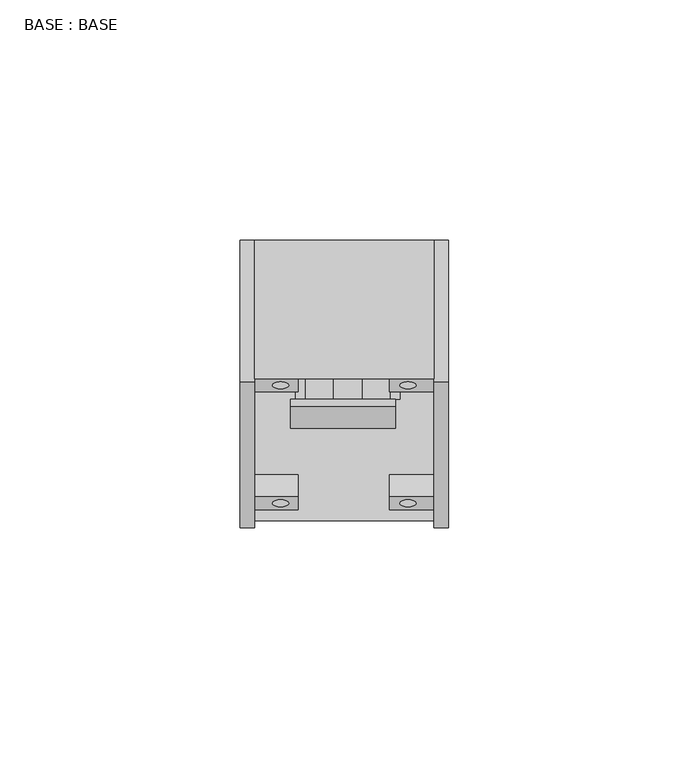
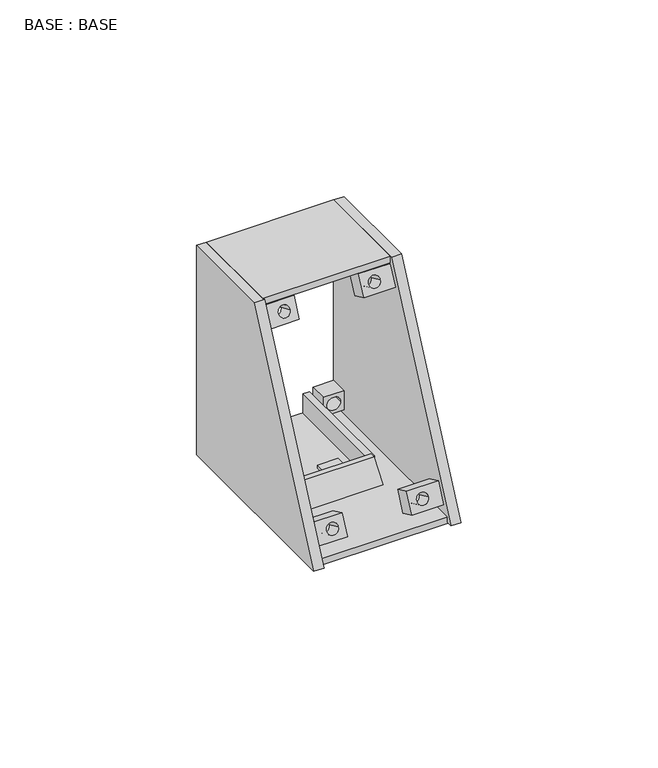
"""IFC4 building model written with IfcOpenShell, lengths in millimetres: proxy geometry, BASE : BASE."""

from ifc_helpers import new_model, si_unit, point, frame, frame_2d, origin, origin_with_axes, place, context, project, spatial, polyline, circle_curve, trimmed, segment, composite_curve, outline, extrude, source, transform, mapped, element, save


def base_base_dd735b77(model_context):
    return source(origin(), model_context, "Body", "SweptSolid", [
        extrude(outline(polyline([(3.2, -2.2), (-3.2, -2.2), (-3.2, 7.1), (3.2, 7.1), (3.2, -2.2)]), holes=[composite_curve([segment(trimmed(circle_curve(frame_2d((0.0, 1.7)), 1.7), [point((0.0, 0.0))], [point((0.0, 3.4))], True, "CARTESIAN"), True, "CONTINUOUS"), segment(trimmed(circle_curve(frame_2d((0.0, 1.7)), 1.7), [point((0.0, 3.4))], [point((0.0, 0.0))], True, "CARTESIAN"), True, "CONTINUOUS")], self_intersect=False)]), frame((2402.2719295, 1326.1385366, 57.7208133), z_axis=(0.0, -0.9063077870366535, 0.4226182617406919), x_axis=(0.0, -0.4226182617406919, -0.9063077870366535)), (0.0, 0.0, 1.0), 5.0),
        extrude(outline(polyline([(3.2, -30.2), (-3.2, -30.2), (-3.2, -21.2), (3.2, -21.2), (3.2, -30.2)]), holes=[composite_curve([segment(trimmed(circle_curve(frame_2d((0.0, -24.8)), 1.7), [point((0.0, -23.1))], [point((0.0, -26.5))], True, "CARTESIAN"), True, "CONTINUOUS"), segment(trimmed(circle_curve(frame_2d((0.0, -24.8)), 1.7), [point((0.0, -26.5))], [point((0.0, -23.1))], True, "CARTESIAN"), True, "CONTINUOUS")], self_intersect=False)]), frame((2402.2719295, 1326.1385366, 57.7208133), z_axis=(0.0, -0.9063077870366535, 0.4226182617406919), x_axis=(0.0, -0.4226182617406919, -0.9063077870366535)), (0.0, 0.0, 1.0), 5.0),
        extrude(outline(polyline([(61.2, -2.2), (54.8, -2.2), (54.8, 7.1), (61.2, 7.1), (61.2, -2.2)]), holes=[composite_curve([segment(trimmed(circle_curve(frame_2d((58.0000001, 1.7)), 1.7), [point((58.0000001, 3.4))], [point((58.0000001, 0.0))], True, "CARTESIAN"), True, "CONTINUOUS"), segment(trimmed(circle_curve(frame_2d((58.0000001, 1.7)), 1.7), [point((58.0000001, 0.0))], [point((58.0000001, 3.4))], True, "CARTESIAN"), True, "CONTINUOUS")], self_intersect=False)]), frame((2402.2719295, 1326.1385366, 57.7208133), z_axis=(0.0, -0.9063077870366535, 0.4226182617406919), x_axis=(0.0, -0.4226182617406919, -0.9063077870366535)), (0.0, 0.0, 1.0), 5.0),
        extrude(outline(polyline([(61.2, -21.2), (61.2, -30.2), (54.8, -30.2), (54.8, -21.2), (61.2, -21.2)]), holes=[composite_curve([segment(trimmed(circle_curve(frame_2d((58.0000001, -24.8)), 1.7), [point((58.0000001, -23.1))], [point((58.0000001, -26.5))], True, "CARTESIAN"), True, "CONTINUOUS"), segment(trimmed(circle_curve(frame_2d((58.0000001, -24.8)), 1.7), [point((58.0000001, -26.5))], [point((58.0000001, -23.1))], True, "CARTESIAN"), True, "CONTINUOUS")], self_intersect=False)]), frame((2402.2719295, 1326.1385366, 57.7208133), z_axis=(0.0, -0.9063077870366535, 0.4226182617406919), x_axis=(0.0, -0.4226182617406919, -0.9063077870366535)), (0.0, 0.0, 1.0), 5.0),
        extrude(outline(polyline([(2394.4431854, 1318.7384159), (2388.4431854, 1318.7384159), (2388.4431854, 1323.7384159), (2394.4431854, 1323.7384159), (2394.4431854, 1318.7384159)])), frame((0.0, 0.0, 6.0), z_axis=(0.0, 0.0, 1.0), x_axis=(1.0, 0.0, 0.0)), (0.0, 0.0, 1.0), 1.0),
        extrude(outline(polyline([(1336.0781618, 2.0), (1344.7384159, 17.0), (1351.7384159, 17.0), (1351.7384159, 15.25), (1346.4884159, 15.25), (1346.4884159, 2.0), (1336.0781618, 2.0)])), frame((2372.0719295, 0.0, 0.0), z_axis=(1.0, 0.0, 0.0), x_axis=(0.0, 1.0, 0.0)), (0.0, 0.0, 1.0), 6.0),
        extrude(outline(polyline([(2409.3719295, 1322.9717492), (2372.0719295, 1322.9717492), (2372.0719295, 1351.7384159), (2409.3719295, 1351.7384159), (2409.3719295, 1322.9717492)])), frame((0.0, 0.0, 63.0), z_axis=(0.0, 0.0, 1.0), x_axis=(1.0, 0.0, 0.0)), (0.0, 0.0, 1.0), 2.0),
        extrude(outline(polyline([(3.0, 2403.3719295), (3.0, 2409.3719295), (9.0, 2409.3719295), (9.0, 2403.3719295), (3.0, 2403.3719295)]), holes=[composite_curve([segment(trimmed(circle_curve(frame_2d((6.0, 2406.3719295)), 2.0), [point((6.0, 2408.3719295))], [point((6.0, 2404.3719295))], True, "CARTESIAN"), True, "CONTINUOUS"), segment(trimmed(circle_curve(frame_2d((6.0, 2406.3719295)), 2.0), [point((6.0, 2404.3719295))], [point((6.0, 2408.3719295))], True, "CARTESIAN"), True, "CONTINUOUS")], self_intersect=False)]), frame((0.0, 1346.4884159, 0.0), z_axis=(0.0, 1.0, 0.0), x_axis=(0.0, 0.0, 1.0)), (0.0, 0.0, 1.0), 5.25),
        extrude(outline(polyline([(3.0, 2378.0719295), (9.0, 2378.0719295), (9.0, 2372.0719295), (3.0, 2372.0719295), (3.0, 2378.0719295)]), holes=[composite_curve([segment(trimmed(circle_curve(frame_2d((6.0, 2375.0719295)), 2.0), [point((6.0, 2377.0719295))], [point((6.0, 2373.0719295))], True, "CARTESIAN"), True, "CONTINUOUS"), segment(trimmed(circle_curve(frame_2d((6.0, 2375.0719295)), 2.0), [point((6.0, 2373.0719295))], [point((6.0, 2377.0719295))], True, "CARTESIAN"), True, "CONTINUOUS")], self_intersect=False)]), frame((0.0, 1346.4884159, 0.0), z_axis=(0.0, 1.0, 0.0), x_axis=(0.0, 0.0, 1.0)), (0.0, 0.0, 1.0), 5.25),
        extrude(outline(polyline([(62.0, 2403.3719295), (56.0, 2403.3719295), (56.0, 2409.3719295), (62.0, 2409.3719295), (62.0, 2403.3719295)]), holes=[composite_curve([segment(trimmed(circle_curve(frame_2d((59.0, 2406.3719295)), 2.0), [point((59.0, 2408.3719295))], [point((59.0, 2404.3719295))], True, "CARTESIAN"), True, "CONTINUOUS"), segment(trimmed(circle_curve(frame_2d((59.0, 2406.3719295)), 2.0), [point((59.0, 2404.3719295))], [point((59.0, 2408.3719295))], True, "CARTESIAN"), True, "CONTINUOUS")], self_intersect=False)]), frame((0.0, 1346.4884159, 0.0), z_axis=(0.0, 1.0, 0.0), x_axis=(0.0, 0.0, 1.0)), (0.0, 0.0, 1.0), 5.25),
        extrude(outline(polyline([(62.0, 2378.0719295), (62.0, 2372.0719295), (56.0, 2372.0719295), (56.0, 2378.0719295), (62.0, 2378.0719295)]), holes=[composite_curve([segment(trimmed(circle_curve(frame_2d((59.0, 2375.0719295)), 2.0), [point((59.0, 2377.0719295))], [point((59.0, 2373.0719295))], True, "CARTESIAN"), True, "CONTINUOUS"), segment(trimmed(circle_curve(frame_2d((59.0, 2375.0719295)), 2.0), [point((59.0, 2373.0719295))], [point((59.0, 2377.0719295))], True, "CARTESIAN"), True, "CONTINUOUS")], self_intersect=False)]), frame((0.0, 1346.4884159, 0.0), z_axis=(0.0, 1.0, 0.0), x_axis=(0.0, 0.0, 1.0)), (0.0, 0.0, 1.0), 5.25),
        extrude(outline(polyline([(1351.7384159, 0.0), (1292.0509228, 0.0), (1322.3609206, 65.0), (1351.7384159, 65.0), (1351.7384159, 0.0)])), frame((2409.3719295, 0.0, 0.0), z_axis=(1.0, 0.0, 0.0), x_axis=(0.0, 1.0, 0.0)), (0.0, 0.0, 1.0), 3.0),
        extrude(outline(polyline([(1351.7384159, 0.0), (1292.0509228, 0.0), (1322.3609206, 65.0), (1351.7384159, 65.0), (1351.7384159, 0.0)])), frame((2369.0719295, 0.0, 0.0), z_axis=(1.0, 0.0, 0.0), x_axis=(0.0, 1.0, 0.0)), (0.0, 0.0, 1.0), 3.0),
        extrude(outline(polyline([(2402.3331854, 1318.7384159), (2400.3331854, 1318.7384159), (2400.3331854, 1351.7384159), (2402.3331854, 1351.7384159), (2402.3331854, 1318.7384159)])), frame((0.0, 0.0, 2.0), z_axis=(0.0, 0.0, 1.0), x_axis=(1.0, 0.0, 0.0)), (0.0, 0.0, 1.0), 6.0),
        extrude(outline(polyline([(2380.5531854, 1318.7384159), (2380.5531854, 1351.7384159), (2382.5531854, 1351.7384159), (2382.5531854, 1318.7384159), (2380.5531854, 1318.7384159)])), frame((0.0, 0.0, 2.0), z_axis=(0.0, 0.0, 1.0), x_axis=(1.0, 0.0, 0.0)), (0.0, 0.0, 1.0), 6.0),
        extrude(outline(polyline([(1318.7384159, 9.0), (1318.7384159, 3.0), (1312.7384159, 3.0), (1317.2253325, 9.0), (1318.7384159, 9.0)])), frame((2379.5519295, 0.0, 0.0), z_axis=(1.0, 0.0, 0.0), x_axis=(0.0, 1.0, 0.0)), (0.0, 0.0, 1.0), 21.78),
        extrude(outline(polyline([(2409.3719295, 1293.4498458), (2372.0719295, 1293.4498458), (2372.0719295, 1351.7384159), (2409.3719295, 1351.7384159), (2409.3719295, 1293.4498458)])), origin_with_axes(), (0.0, 0.0, 1.0), 2.0),
    ])


if __name__ == "__main__":
    model = new_model("IFC4")
    model_context = context("Model", 3, world=origin())
    ifc_project = project(units=[si_unit("LENGTHUNIT", "METRE", prefix="MILLI")], contexts=[model_context])
    site = spatial("IfcSite", under=ifc_project)
    building = spatial("IfcBuilding", under=site)
    placement = place(None, origin())
    base_base_shape = base_base_dd735b77(model_context)
    element("IfcBuildingElementProxy", 1, Name="BASE : BASE", ObjectType="BASE : BASE", at=placement, inside=building, context=model_context, shape_type="MappedRepresentation", body=[
        mapped(base_base_shape, transform((0.0, 0.0, 0.0), x_axis=(1.0, 0.0, 0.0), y_axis=(0.0, 1.0, 0.0), z_axis=(0.0, 0.0, 1.0))),
    ])
    save(model, "model.ifc")

# Revit data of these elements
# Project information
#   Data de emissão do projeto = "Data de emissão"
#   Status do projeto = "Status do projeto"
#   Nome do cliente = "Proprietário"
#   Endereço do projeto = "Insira aqui o endereço"
#   Nome do projeto = "Nome do projeto"
#   Número do projeto = "0001"
# Element 1 (IfcBuildingElementProxy, "BASE : BASE")
#   Materials on its faces: ".BOX LATERAL"
# Materials
#   ".BOX LATERAL": class "Vidro", colour RGB 236 240 239, transparency 0.15, Cost = 0
